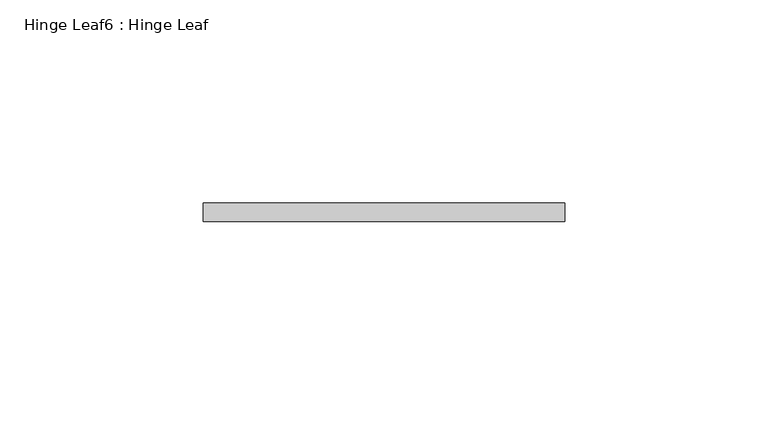
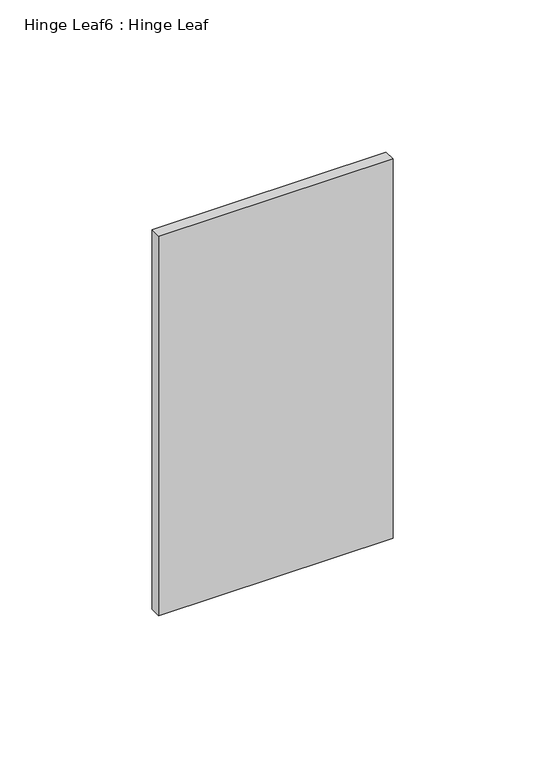
"""IFC4 building model written with IfcOpenShell, lengths in millimetres: proxy geometry, Hinge Leaf6 : Hinge Leaf."""

import ifcopenshell
import ifcopenshell.guid

model = None  # the IFC model being written
_history = None  # IfcOwnerHistory: only IFC2X3 demands one
_inside = {}  # id of a spatial element -> (the spatial element, [elements in it])
_under = {}  # id of a project, library or spatial element -> (it, [spatial elements below it])
_declared = {}  # id of a project -> (the project, [libraries it declares])
_typed = {}  # id of a type object -> (the type object, [elements of that type])
_made_of = {}  # id of a material, layer set ... -> (it, [elements and type objects made of it])


def new_model(schema):
    """Start an empty IFC model of exactly this schema.

    Asked for "IFC4X3", IfcOpenShell would pick the latest addendum, in which some entities
    have other attributes; the version numbers below select the first issue.
    IFC2X3 requires an IfcOwnerHistory on every rooted entity: one is made here for all.
    """
    global model, _history
    if schema == "IFC4X3":
        model = ifcopenshell.file(schema_version=(4, 3, 0, 0))
    else:
        model = ifcopenshell.file(schema=schema)
    _inside.clear()
    _under.clear()
    _declared.clear()
    _typed.clear()
    _made_of.clear()
    _history = None
    if model.schema == "IFC2X3":
        org = make("IfcOrganization", Name="unknown")
        user = make(
            "IfcPersonAndOrganization",
            ThePerson=make("IfcPerson", FamilyName="unknown"),
            TheOrganization=org,
        )
        app = make(
            "IfcApplication",
            ApplicationDeveloper=org,
            Version="unknown",
            ApplicationFullName="unknown",
            ApplicationIdentifier="unknown",
        )
        _history = make(
            "IfcOwnerHistory",
            OwningUser=user,
            OwningApplication=app,
            ChangeAction="ADDED",
            CreationDate=0,
        )
    return model


def make(cls, **values):
    """One entity of the class cls with the attributes given. An attribute that is None is left unset."""
    return model.create_entity(
        cls, **{name: value for name, value in values.items() if value is not None}
    )


def rooted(cls, **values):
    """An entity with a GlobalId (a new one), such as an element, a storey or a relation."""
    return make(cls, GlobalId=ifcopenshell.guid.new(), OwnerHistory=_history, **values)


def si_unit(unit_type, name, prefix=None):
    """IfcSIUnit, for example si_unit("LENGTHUNIT", "METRE", prefix="MILLI")."""
    return make("IfcSIUnit", UnitType=unit_type, Prefix=prefix, Name=name)


def assignment(units):
    """IfcUnitAssignment: the units of a project."""
    return None if units is None else make("IfcUnitAssignment", Units=units)


def point(xyz):
    """IfcCartesianPoint."""
    return None if xyz is None else make("IfcCartesianPoint", Coordinates=xyz)


def direction(xyz):
    """IfcDirection."""
    return None if xyz is None else make("IfcDirection", DirectionRatios=xyz)


def frame(location, z_axis=None, x_axis=None):
    """IfcAxis2Placement3D, a coordinate frame: its origin and axes. An axis left out is left unset."""
    return make(
        "IfcAxis2Placement3D",
        Location=point(location),
        Axis=direction(z_axis),
        RefDirection=direction(x_axis),
    )


def origin():
    """The frame at (0, 0, 0) with its axes left unset."""
    return frame((0.0, 0.0, 0.0))


def place(relative_to, where):
    """IfcLocalPlacement: puts the frame where relative to a parent placement (None: the world)."""
    return make(
        "IfcLocalPlacement", PlacementRelTo=relative_to, RelativePlacement=where
    )


def context(
    kind, dimensions, precision=None, world=None, true_north=None, identifier=None
):
    """IfcGeometricRepresentationContext, for example the 3D "Model" context."""
    return make(
        "IfcGeometricRepresentationContext",
        ContextIdentifier=identifier,
        ContextType=kind,
        CoordinateSpaceDimension=dimensions,
        Precision=precision,
        WorldCoordinateSystem=world,
        TrueNorth=true_north,
    )


def project(units=None, contexts=None):
    """IfcProject with its units and contexts."""
    return rooted(
        "IfcProject",
        Name="project",
        RepresentationContexts=contexts,
        UnitsInContext=assignment(units),
    )


def spatial(cls, under=None, at=None, **own):
    """A site, building, storey or space (cls), placed at a placement, below another one or the project."""
    s = rooted(cls, ObjectPlacement=at, **own)
    if under is not None:
        _under.setdefault(under.id(), (under, []))[1].append(s)
    return s


def polyline(points):
    """IfcPolyline through the points."""
    return make("IfcPolyline", Points=[point(p) for p in points])


def outline(outer, holes=None, kind="AREA"):
    """IfcArbitraryClosedProfileDef: a profile drawn as a closed curve; with holes, ...WithVoids."""
    if holes is None:
        return make("IfcArbitraryClosedProfileDef", ProfileType=kind, OuterCurve=outer)
    return make(
        "IfcArbitraryProfileDefWithVoids",
        ProfileType=kind,
        OuterCurve=outer,
        InnerCurves=holes,
    )


def extrude(swept, where, along, depth):
    """IfcExtrudedAreaSolid: the profile swept, set in the frame where, extruded along a direction by depth."""
    return make(
        "IfcExtrudedAreaSolid",
        SweptArea=swept,
        Position=where,
        ExtrudedDirection=direction(along),
        Depth=depth,
    )


def shape(context_of_items, identifier, shape_type, items):
    """IfcShapeRepresentation: the items that make up one representation, for example the "Body"."""
    return make(
        "IfcShapeRepresentation",
        ContextOfItems=context_of_items,
        RepresentationIdentifier=identifier,
        RepresentationType=shape_type,
        Items=items,
    )


def source(mapping_origin, context_of_items, identifier, shape_type, items):
    """IfcRepresentationMap: a shape defined once, which mapped items show again and again."""
    return make(
        "IfcRepresentationMap",
        MappingOrigin=mapping_origin,
        MappedRepresentation=shape(context_of_items, identifier, shape_type, items),
    )


def transform(
    local_origin,
    x_axis=None,
    y_axis=None,
    z_axis=None,
    scale=None,
    scale2=None,
    scale3=None,
    uniform=True,
):
    """IfcCartesianTransformationOperator3D, or its non-uniform kind. x_axis, y_axis, z_axis: its Axis1, 2, 3."""
    if uniform:
        return make(
            "IfcCartesianTransformationOperator3D",
            Axis1=direction(x_axis),
            Axis2=direction(y_axis),
            LocalOrigin=point(local_origin),
            Scale=scale,
            Axis3=direction(z_axis),
        )
    return make(
        "IfcCartesianTransformationOperator3DnonUniform",
        Axis1=direction(x_axis),
        Axis2=direction(y_axis),
        LocalOrigin=point(local_origin),
        Scale=scale,
        Axis3=direction(z_axis),
        Scale2=scale2,
        Scale3=scale3,
    )


def mapped(mapping_source, mapping_target):
    """IfcMappedItem: shows the shape of a source again, moved by a transform."""
    return make(
        "IfcMappedItem", MappingSource=mapping_source, MappingTarget=mapping_target
    )


def made_of(thing, what):
    """Note that an element or type object is made of a material, layer set ...; save() writes the relation."""
    if what is not None:
        _made_of.setdefault(what.id(), (what, []))[1].append(thing)
    return thing


def element(
    cls,
    number,
    at=None,
    inside=None,
    cuts=None,
    type_object=None,
    material=None,
    context=None,
    identifier="Body",
    shape_type=None,
    held_by="IfcProductDefinitionShape",
    body=None,
    shapes=None,
    **own,
):
    """One element of the class cls, such as IfcWall. Its Tag is "e" and its number.

    at: its placement. inside: the storey or other place that contains it. cuts: it is an
    opening in that element (IfcRelVoidsElement). A single representation is given by context,
    identifier, shape_type and body (its items); several are given by shapes. held_by: the class
    of the entity that holds the representations. save() writes the other relations.
    """
    e = rooted(cls, Tag="e%d" % number, ObjectPlacement=at, **own)
    if body is not None:
        shapes = [shape(context, identifier, shape_type, body)]
    if shapes is not None:
        e.Representation = make(held_by, Representations=shapes)
    if inside is not None:
        _inside.setdefault(inside.id(), (inside, []))[1].append(e)
    if cuts is not None:
        rooted(
            "IfcRelVoidsElement", RelatingBuildingElement=cuts, RelatedOpeningElement=e
        )
    if type_object is not None:
        _typed.setdefault(type_object.id(), (type_object, []))[1].append(e)
    return made_of(e, material)


def aggregate(whole, parts):
    """IfcRelAggregates: a whole, such as a stair, and the parts it consists of."""
    return rooted("IfcRelAggregates", RelatingObject=whole, RelatedObjects=parts)


def save(model, path):
    """Write the relations noted so far, then the file.

    IfcRelAggregates (storeys below a building ...), IfcRelContainedInSpatialStructure (elements
    in a storey), IfcRelDefinesByType, IfcRelAssociatesMaterial and IfcRelDeclares: one each for
    every whole, place, type object, material and project.
    """
    for whole, parts in _under.values():
        aggregate(whole, parts)
    for where, things in _inside.values():
        rooted(
            "IfcRelContainedInSpatialStructure",
            RelatedElements=things,
            RelatingStructure=where,
        )
    for kind, things in _typed.values():
        rooted("IfcRelDefinesByType", RelatedObjects=things, RelatingType=kind)
    for what, things in _made_of.values():
        rooted("IfcRelAssociatesMaterial", RelatedObjects=things, RelatingMaterial=what)
    for by, libraries in _declared.values():
        rooted("IfcRelDeclares", RelatingContext=by, RelatedDefinitions=libraries)
    model.write(path)


def hinge_leaf6_hinge_leaf_bcfbb292(model_context):
    return source(origin(), model_context, "Body", "SweptSolid", [
        extrude(outline(polyline([(587327.7934739, -533980.5883841), (587327.7934739, -533976.0163841), (587416.6934739, -533976.0163841), (587416.6934739, -533980.5883841), (587327.7934739, -533980.5883841)])), frame((0.0, 0.0, 311.15), z_axis=(0.0, 0.0, 1.0), x_axis=(1.0, 0.0, 0.0)), (0.0, 0.0, 1.0), 152.4),
    ])


if __name__ == "__main__":
    model = new_model("IFC4")
    model_context = context("Model", 3, world=origin())
    ifc_project = project(units=[si_unit("LENGTHUNIT", "METRE", prefix="MILLI")], contexts=[model_context])
    site = spatial("IfcSite", under=ifc_project)
    building = spatial("IfcBuilding", under=site)
    placement = place(None, origin())
    hinge_leaf6_hinge_leaf_shape = hinge_leaf6_hinge_leaf_bcfbb292(model_context)
    element("IfcBuildingElementProxy", 1, Name="Hinge Leaf6 : Hinge Leaf", ObjectType="Hinge Leaf6 : Hinge Leaf", at=placement, inside=building, context=model_context, shape_type="MappedRepresentation", body=[
        mapped(hinge_leaf6_hinge_leaf_shape, transform((0.0, 0.0, 0.0), x_axis=(1.0, 0.0, 0.0), y_axis=(0.0, 1.0, 0.0), z_axis=(0.0, 0.0, 1.0))),
    ])
    save(model, "model.ifc")

# Revit data of these elements
# Element 1 (IfcBuildingElementProxy, "Hinge Leaf6 : Hinge Leaf")
#   Materials on its faces: "6\"X6\" WELD-ON STL BUTT HINGE"
# Materials
#   "6\"X6\" WELD-ON STL BUTT HINGE": class "Metal", colour RGB 189 187 185, transparency 0, Description = "Carbon steel", Cost = 0
